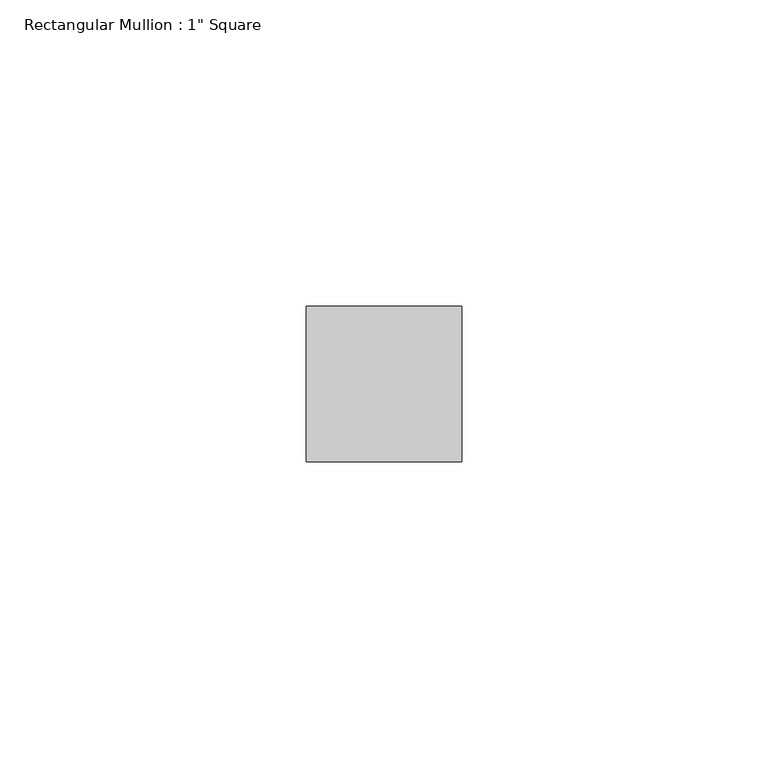
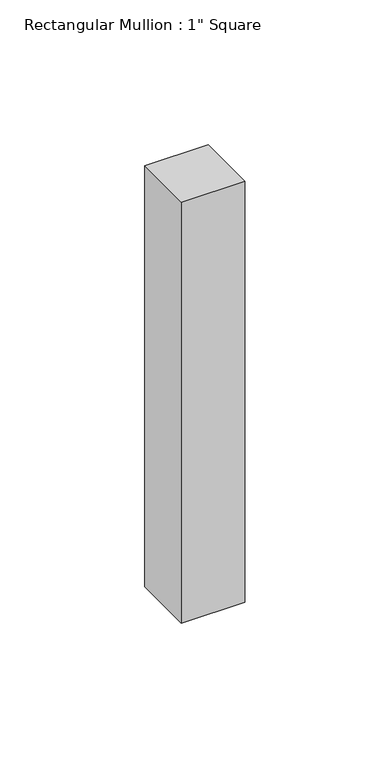
"""IFC4 building model written with IfcOpenShell, lengths in millimetres: member geometry."""

import ifcopenshell
import ifcopenshell.guid

model = None  # the IFC model being written
_history = None  # IfcOwnerHistory: only IFC2X3 demands one
_inside = {}  # id of a spatial element -> (the spatial element, [elements in it])
_under = {}  # id of a project, library or spatial element -> (it, [spatial elements below it])
_declared = {}  # id of a project -> (the project, [libraries it declares])
_typed = {}  # id of a type object -> (the type object, [elements of that type])
_made_of = {}  # id of a material, layer set ... -> (it, [elements and type objects made of it])


def new_model(schema):
    """Start an empty IFC model of exactly this schema.

    Asked for "IFC4X3", IfcOpenShell would pick the latest addendum, in which some entities
    have other attributes; the version numbers below select the first issue.
    IFC2X3 requires an IfcOwnerHistory on every rooted entity: one is made here for all.
    """
    global model, _history
    if schema == "IFC4X3":
        model = ifcopenshell.file(schema_version=(4, 3, 0, 0))
    else:
        model = ifcopenshell.file(schema=schema)
    _inside.clear()
    _under.clear()
    _declared.clear()
    _typed.clear()
    _made_of.clear()
    _history = None
    if model.schema == "IFC2X3":
        org = make("IfcOrganization", Name="unknown")
        user = make(
            "IfcPersonAndOrganization",
            ThePerson=make("IfcPerson", FamilyName="unknown"),
            TheOrganization=org,
        )
        app = make(
            "IfcApplication",
            ApplicationDeveloper=org,
            Version="unknown",
            ApplicationFullName="unknown",
            ApplicationIdentifier="unknown",
        )
        _history = make(
            "IfcOwnerHistory",
            OwningUser=user,
            OwningApplication=app,
            ChangeAction="ADDED",
            CreationDate=0,
        )
    return model


def make(cls, **values):
    """One entity of the class cls with the attributes given. An attribute that is None is left unset."""
    return model.create_entity(
        cls, **{name: value for name, value in values.items() if value is not None}
    )


def rooted(cls, **values):
    """An entity with a GlobalId (a new one), such as an element, a storey or a relation."""
    return make(cls, GlobalId=ifcopenshell.guid.new(), OwnerHistory=_history, **values)


def si_unit(unit_type, name, prefix=None):
    """IfcSIUnit, for example si_unit("LENGTHUNIT", "METRE", prefix="MILLI")."""
    return make("IfcSIUnit", UnitType=unit_type, Prefix=prefix, Name=name)


def assignment(units):
    """IfcUnitAssignment: the units of a project."""
    return None if units is None else make("IfcUnitAssignment", Units=units)


def point(xyz):
    """IfcCartesianPoint."""
    return None if xyz is None else make("IfcCartesianPoint", Coordinates=xyz)


def direction(xyz):
    """IfcDirection."""
    return None if xyz is None else make("IfcDirection", DirectionRatios=xyz)


def frame(location, z_axis=None, x_axis=None):
    """IfcAxis2Placement3D, a coordinate frame: its origin and axes. An axis left out is left unset."""
    return make(
        "IfcAxis2Placement3D",
        Location=point(location),
        Axis=direction(z_axis),
        RefDirection=direction(x_axis),
    )


def origin():
    """The frame at (0, 0, 0) with its axes left unset."""
    return frame((0.0, 0.0, 0.0))


def place(relative_to, where):
    """IfcLocalPlacement: puts the frame where relative to a parent placement (None: the world)."""
    return make(
        "IfcLocalPlacement", PlacementRelTo=relative_to, RelativePlacement=where
    )


def context(
    kind, dimensions, precision=None, world=None, true_north=None, identifier=None
):
    """IfcGeometricRepresentationContext, for example the 3D "Model" context."""
    return make(
        "IfcGeometricRepresentationContext",
        ContextIdentifier=identifier,
        ContextType=kind,
        CoordinateSpaceDimension=dimensions,
        Precision=precision,
        WorldCoordinateSystem=world,
        TrueNorth=true_north,
    )


def project(units=None, contexts=None):
    """IfcProject with its units and contexts."""
    return rooted(
        "IfcProject",
        Name="project",
        RepresentationContexts=contexts,
        UnitsInContext=assignment(units),
    )


def spatial(cls, under=None, at=None, **own):
    """A site, building, storey or space (cls), placed at a placement, below another one or the project."""
    s = rooted(cls, ObjectPlacement=at, **own)
    if under is not None:
        _under.setdefault(under.id(), (under, []))[1].append(s)
    return s


def polyline(points):
    """IfcPolyline through the points."""
    return make("IfcPolyline", Points=[point(p) for p in points])


def outline(outer, holes=None, kind="AREA"):
    """IfcArbitraryClosedProfileDef: a profile drawn as a closed curve; with holes, ...WithVoids."""
    if holes is None:
        return make("IfcArbitraryClosedProfileDef", ProfileType=kind, OuterCurve=outer)
    return make(
        "IfcArbitraryProfileDefWithVoids",
        ProfileType=kind,
        OuterCurve=outer,
        InnerCurves=holes,
    )


def extrude(swept, where, along, depth):
    """IfcExtrudedAreaSolid: the profile swept, set in the frame where, extruded along a direction by depth."""
    return make(
        "IfcExtrudedAreaSolid",
        SweptArea=swept,
        Position=where,
        ExtrudedDirection=direction(along),
        Depth=depth,
    )


def shape(context_of_items, identifier, shape_type, items):
    """IfcShapeRepresentation: the items that make up one representation, for example the "Body"."""
    return make(
        "IfcShapeRepresentation",
        ContextOfItems=context_of_items,
        RepresentationIdentifier=identifier,
        RepresentationType=shape_type,
        Items=items,
    )


def source(mapping_origin, context_of_items, identifier, shape_type, items):
    """IfcRepresentationMap: a shape defined once, which mapped items show again and again."""
    return make(
        "IfcRepresentationMap",
        MappingOrigin=mapping_origin,
        MappedRepresentation=shape(context_of_items, identifier, shape_type, items),
    )


def transform(
    local_origin,
    x_axis=None,
    y_axis=None,
    z_axis=None,
    scale=None,
    scale2=None,
    scale3=None,
    uniform=True,
):
    """IfcCartesianTransformationOperator3D, or its non-uniform kind. x_axis, y_axis, z_axis: its Axis1, 2, 3."""
    if uniform:
        return make(
            "IfcCartesianTransformationOperator3D",
            Axis1=direction(x_axis),
            Axis2=direction(y_axis),
            LocalOrigin=point(local_origin),
            Scale=scale,
            Axis3=direction(z_axis),
        )
    return make(
        "IfcCartesianTransformationOperator3DnonUniform",
        Axis1=direction(x_axis),
        Axis2=direction(y_axis),
        LocalOrigin=point(local_origin),
        Scale=scale,
        Axis3=direction(z_axis),
        Scale2=scale2,
        Scale3=scale3,
    )


def mapped(mapping_source, mapping_target):
    """IfcMappedItem: shows the shape of a source again, moved by a transform."""
    return make(
        "IfcMappedItem", MappingSource=mapping_source, MappingTarget=mapping_target
    )


def made_of(thing, what):
    """Note that an element or type object is made of a material, layer set ...; save() writes the relation."""
    if what is not None:
        _made_of.setdefault(what.id(), (what, []))[1].append(thing)
    return thing


def element(
    cls,
    number,
    at=None,
    inside=None,
    cuts=None,
    type_object=None,
    material=None,
    context=None,
    identifier="Body",
    shape_type=None,
    held_by="IfcProductDefinitionShape",
    body=None,
    shapes=None,
    **own,
):
    """One element of the class cls, such as IfcWall. Its Tag is "e" and its number.

    at: its placement. inside: the storey or other place that contains it. cuts: it is an
    opening in that element (IfcRelVoidsElement). A single representation is given by context,
    identifier, shape_type and body (its items); several are given by shapes. held_by: the class
    of the entity that holds the representations. save() writes the other relations.
    """
    e = rooted(cls, Tag="e%d" % number, ObjectPlacement=at, **own)
    if body is not None:
        shapes = [shape(context, identifier, shape_type, body)]
    if shapes is not None:
        e.Representation = make(held_by, Representations=shapes)
    if inside is not None:
        _inside.setdefault(inside.id(), (inside, []))[1].append(e)
    if cuts is not None:
        rooted(
            "IfcRelVoidsElement", RelatingBuildingElement=cuts, RelatedOpeningElement=e
        )
    if type_object is not None:
        _typed.setdefault(type_object.id(), (type_object, []))[1].append(e)
    return made_of(e, material)


def aggregate(whole, parts):
    """IfcRelAggregates: a whole, such as a stair, and the parts it consists of."""
    return rooted("IfcRelAggregates", RelatingObject=whole, RelatedObjects=parts)


def save(model, path):
    """Write the relations noted so far, then the file.

    IfcRelAggregates (storeys below a building ...), IfcRelContainedInSpatialStructure (elements
    in a storey), IfcRelDefinesByType, IfcRelAssociatesMaterial and IfcRelDeclares: one each for
    every whole, place, type object, material and project.
    """
    for whole, parts in _under.values():
        aggregate(whole, parts)
    for where, things in _inside.values():
        rooted(
            "IfcRelContainedInSpatialStructure",
            RelatedElements=things,
            RelatingStructure=where,
        )
    for kind, things in _typed.values():
        rooted("IfcRelDefinesByType", RelatedObjects=things, RelatingType=kind)
    for what, things in _made_of.values():
        rooted("IfcRelAssociatesMaterial", RelatedObjects=things, RelatingMaterial=what)
    for by, libraries in _declared.values():
        rooted("IfcRelDeclares", RelatingContext=by, RelatedDefinitions=libraries)
    model.write(path)


def member_fda38710(model_context):
    return source(origin(), model_context, "Body", "SweptSolid", [
        extrude(outline(polyline([(0.0, 12.7), (0.0, -12.7), (-25.4, -12.7), (-25.4, 12.7), (0.0, 12.7)])), frame((0.0, 0.0, -177.8), z_axis=(0.0, 0.0, 1.0), x_axis=(1.0, 0.0, 0.0)), (0.0, 0.0, 1.0), 177.8),
    ])


if __name__ == "__main__":
    model = new_model("IFC4")
    model_context = context("Model", 3, world=origin())
    ifc_project = project(units=[si_unit("LENGTHUNIT", "METRE", prefix="MILLI")], contexts=[model_context])
    site = spatial("IfcSite", under=ifc_project)
    building = spatial("IfcBuilding", under=site)
    placement = place(None, origin())
    member_shape = member_fda38710(model_context)
    element("IfcMember", 1, ObjectType="Rectangular Mullion : 1\" Square", at=placement, inside=building, context=model_context, shape_type="MappedRepresentation", body=[
        mapped(member_shape, transform((0.0, 0.0, 0.0), x_axis=(1.0, 0.0, 0.0), y_axis=(0.0, 1.0, 0.0), z_axis=(0.0, 0.0, 1.0))),
    ])
    save(model, "model.ifc")

# Revit data of these elements
# Type "Rectangular Mullion : 1\" Square"
#   built-in parameter 1007304 = 0.0833333 (stored number, unit not read)
#   built-in parameter 1007301 = 0.0416667 (stored number, unit not read)
#   built-in parameter 1007300 = 0.0416667 (stored number, unit not read)
# Element 1 (IfcMember, "Rectangular Mullion : 1\" Square")
#   Materials on its faces: "Metal - Aluminum"
# Materials
#   "Metal - Aluminum": class "Metal", colour RGB 247 247 247, transparency 0
